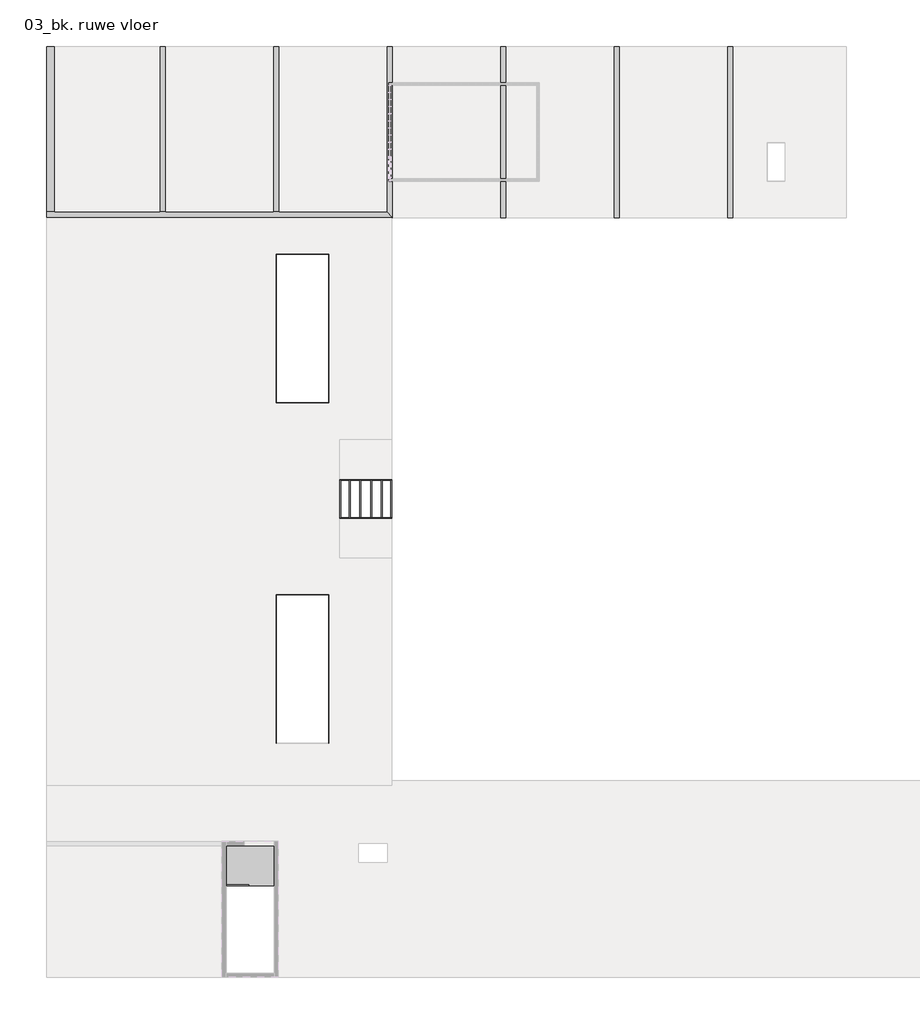
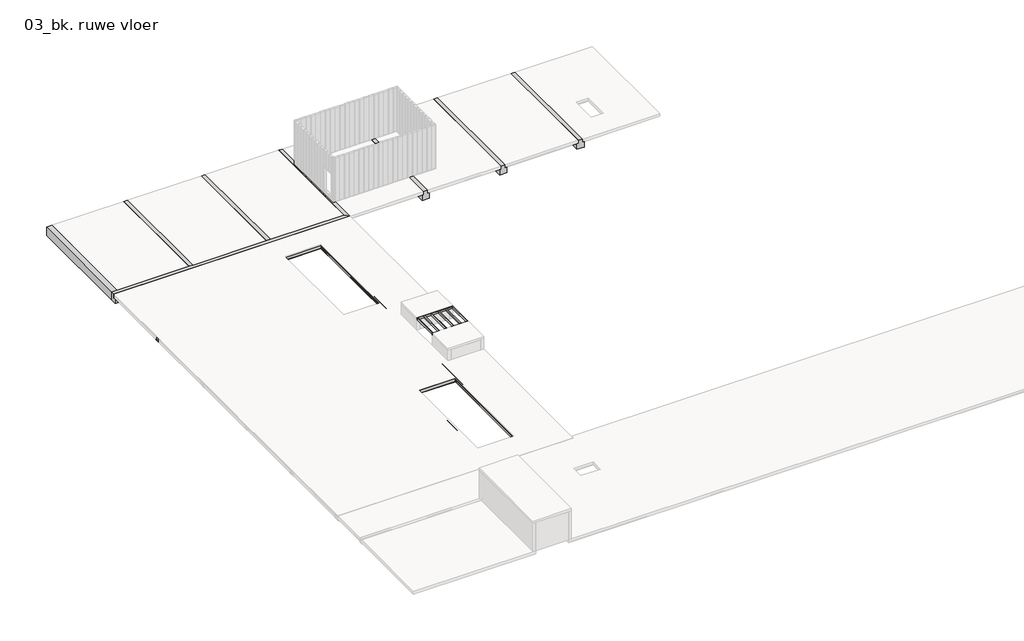
# One storey, part 9 of 9: 26 beams, 1 proxy.
# Revit data of these elements (continued)
# Element 20 (IfcBeam, "NLRS_28_SF_LIB_stalen ligger HEB-AV-CWV-MMBS-SRP_gen_rsf : stalen ligger_gen__HEB 260")
#   IfcGUID = "13lTCcCQ95UOWcvnmPh7D7"
#   Comments = ""
#   NLRS_C_lengte = 12698 mm
#   IsExternal = yes
#   LoadBearing = yes
#   Phase Created = NLRS_nieuw
#   Materials on its faces: "NLRS_h2_staal_gen_rsf"
# Element 21 (IfcBeam, "NLRS_28_SF_LIB_stalen ligger HEB-AV-CWV-MMBS-SRP_gen_rsf : stalen ligger_gen__HEB 260")
#   IfcGUID = "13lTCcCQ95UOWcvnmPh7D_"
#   Comments = ""
#   NLRS_C_lengte = 12637.5 mm
#   IsExternal = yes
#   LoadBearing = yes
#   Phase Created = NLRS_nieuw
#   Materials on its faces: "NLRS_h2_staal_gen_rsf"
# Element 22 (IfcBeam, "NLRS_28_SF_LIB_stalen ligger HEB-AV-CWV-MMBS-SRP_gen_rsf : stalen ligger_gen__HEB 260")
#   IfcGUID = "13lTCcCQ95UOWcvnmPh7Du"
#   Comments = ""
#   NLRS_C_lengte = 12637.5 mm
#   IsExternal = yes
#   LoadBearing = yes
#   Phase Created = NLRS_nieuw
#   Materials on its faces: "NLRS_h2_staal_gen_rsf"
# Element 23 (IfcBeam, "NLRS_28_SF_LIB_houten balk-MMBW-SRP_gen_rsf : houten balk_gen__bxh 58x156")
#   IfcGUID = "3PFmhy1jzBXho9jMrHR5Eo"
#   NLRS_C_lengte = 2250 mm
#   IsExternal = yes
#   LoadBearing = yes
#   Phase Created = NLRS_nieuw
#   Materials on its faces: "NLRS_i2_hout naaldhout vuren_gen_rsf"
# Element 24 (IfcBeam, "NLRS_28_SF_LIB_houten balk-MMBW-SRP_gen_rsf : houten balk_gen__bxh 58x156")
#   IfcGUID = "3PFmhy1jzBXho9jMrHR5Em"
#   NLRS_C_lengte = 2250 mm
#   IsExternal = yes
#   LoadBearing = yes
#   Phase Created = NLRS_nieuw
#   Materials on its faces: "NLRS_i2_hout naaldhout vuren_gen_rsf"
# Element 25 (IfcBeam, "NLRS_28_SF_LIB_houten balk-MMBW-SRP_gen_rsf : houten balk_gen__bxh 58x156")
#   IfcGUID = "3PFmhy1jzBXho9jMrHR5E_"
#   NLRS_C_lengte = 2250 mm
#   IsExternal = yes
#   LoadBearing = yes
#   Phase Created = NLRS_nieuw
#   Materials on its faces: "NLRS_i2_hout naaldhout vuren_gen_rsf"
# Element 26 (IfcBeam, "NLRS_28_SF_LIB_houten balk-MMBW-SRP_gen_rsf : houten balk_gen__bxh 58x156")
#   IfcGUID = "3PFmhy1jzBXho9jMrHR5Ey"
#   NLRS_C_lengte = 2250 mm
#   IsExternal = yes
#   LoadBearing = yes
#   Phase Created = NLRS_nieuw
#   Materials on its faces: "NLRS_i2_hout naaldhout vuren_gen_rsf"
# Element 27 (IfcBuildingElementProxy, "NLRS_24_GM_UN_rechthoekig bordes prefab zonder oplegnok-AV_gen_rsf : prefab bordes_gen__2300x2730")
#   IfcGUID = "2CEqVLPNH8KRN7ghwV3apU"
#   IsExternal = no
#   LoadBearing = yes
#   Phase Created = NLRS_nieuw
#   Materials on its faces: "NLRS_f2_beton prefab_gen_rsf"
# Materials
#   "NLRS_f2_beton prefab_gen_rsf": class "F - Niet gebakken kunststeen", colour RGB 129 133 118, transparency 0, Keynote = "f2", Manufacturer = "Revit Standards Foundation", URL = "www.revitstandards.org", Description = "beton prefab", Cost = 0
#   "NLRS_i2_hout naaldhout vuren_gen_rsf": class "I - Hout", colour RGB 234 199 147, transparency 0, Keynote = "i2", Manufacturer = "Revit Standards Foundation", URL = "www.revitstandards.org", Description = "hout vuren", Cost = 0
#   "NLRS_h2_staal_gen_rsf": class "H - Metaal", colour RGB 189 187 185, transparency 0, Keynote = "h2", Manufacturer = "Revit Standards Foundation", URL = "www.revitstandards.org", Description = "staal", Cost = 0
